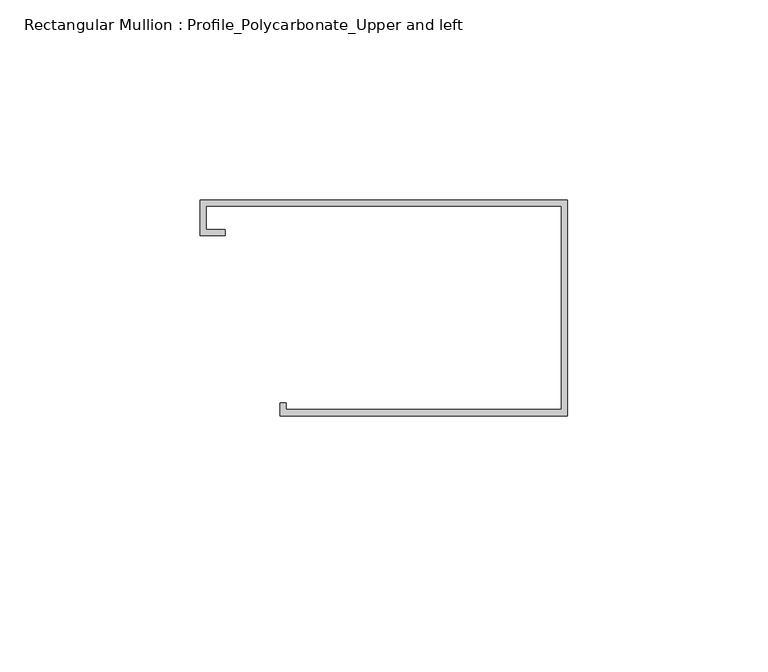
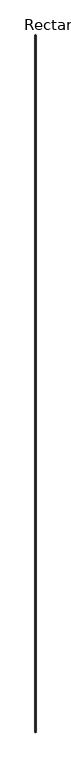
"""IFC4 building model written with IfcOpenShell, lengths in millimetres: member geometry, Rectangular Mullion : Profile_Polycarbonate_Upper and left."""

from ifc_helpers import new_model, si_unit, frame, origin, place, context, project, spatial, polyline, outline, extrude, source, transform, mapped, element, save


def rectangular_mullion_profile_polycarbonate_upper_and_left_6c0196e8(model_context):
    return source(origin(), model_context, "Body", "SweptSolid", [
        extrude(outline(polyline([(0.0, 28.984575), (0.0, -25.015825), (-71.9836, -25.015825), (-71.9836, -21.840825), (-70.3961, -21.840825), (-70.3961, -23.428325), (-1.5875, -23.428325), (-1.5875, 27.397075), (-90.4113, 27.397075), (-90.4113, 21.580475), (-85.6488, 21.580475), (-85.6488, 19.992975), (-91.9988, 19.992975), (-91.9988, 28.984575), (0.0, 28.984575)])), frame((0.0, 0.0, -80917.7063063), z_axis=(0.0, 0.0, 1.0), x_axis=(1.0, 0.0, 0.0)), (0.0, 0.0, 1.0), 80917.7063063),
    ])


if __name__ == "__main__":
    model = new_model("IFC4")
    model_context = context("Model", 3, world=origin())
    ifc_project = project(units=[si_unit("LENGTHUNIT", "METRE", prefix="MILLI")], contexts=[model_context])
    site = spatial("IfcSite", under=ifc_project)
    building = spatial("IfcBuilding", under=site)
    placement = place(None, origin())
    rectangular_mullion_profile_polycarbonate_upper_and_left_shape = rectangular_mullion_profile_polycarbonate_upper_and_left_6c0196e8(model_context)
    element("IfcMember", 1, ObjectType="Rectangular Mullion : Profile_Polycarbonate_Upper and left", at=placement, inside=building, context=model_context, shape_type="MappedRepresentation", body=[
        mapped(rectangular_mullion_profile_polycarbonate_upper_and_left_shape, transform((0.0, 0.0, 0.0), x_axis=(1.0, 0.0, 0.0), y_axis=(0.0, 1.0, 0.0), z_axis=(0.0, 0.0, 1.0))),
    ])
    save(model, "model.ifc")

# Revit data of these elements
# Type "Rectangular Mullion : Profile_Polycarbonate_Upper and left"
#   built-in parameter 1007322 = 0.177167 (stored number, unit not read)
#   built-in parameter 1007321 = 0.00520833 (stored number, unit not read)
#   built-in parameter 1007320 = 0 (stored number, unit not read)
